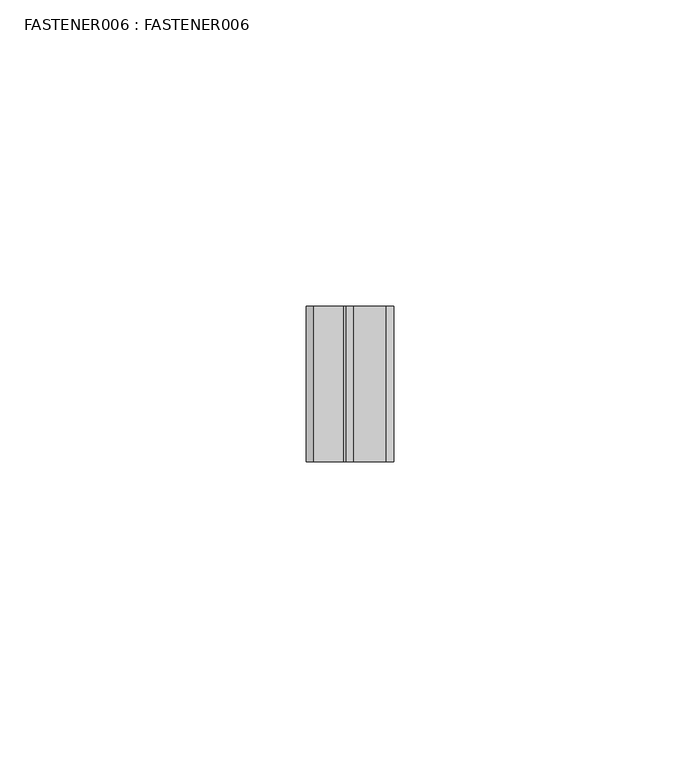
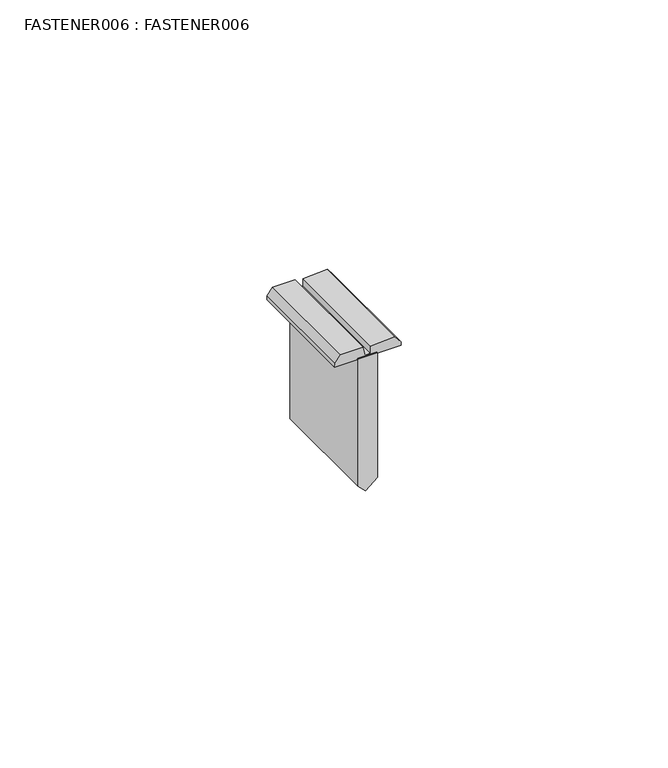
"""IFC4 building model written with IfcOpenShell, lengths in millimetres: proxy geometry, FASTENER006 : FASTENER006."""

import ifcopenshell
import ifcopenshell.guid

model = None  # the IFC model being written
_history = None  # IfcOwnerHistory: only IFC2X3 demands one
_inside = {}  # id of a spatial element -> (the spatial element, [elements in it])
_under = {}  # id of a project, library or spatial element -> (it, [spatial elements below it])
_declared = {}  # id of a project -> (the project, [libraries it declares])
_typed = {}  # id of a type object -> (the type object, [elements of that type])
_made_of = {}  # id of a material, layer set ... -> (it, [elements and type objects made of it])


def new_model(schema):
    """Start an empty IFC model of exactly this schema.

    Asked for "IFC4X3", IfcOpenShell would pick the latest addendum, in which some entities
    have other attributes; the version numbers below select the first issue.
    IFC2X3 requires an IfcOwnerHistory on every rooted entity: one is made here for all.
    """
    global model, _history
    if schema == "IFC4X3":
        model = ifcopenshell.file(schema_version=(4, 3, 0, 0))
    else:
        model = ifcopenshell.file(schema=schema)
    _inside.clear()
    _under.clear()
    _declared.clear()
    _typed.clear()
    _made_of.clear()
    _history = None
    if model.schema == "IFC2X3":
        org = make("IfcOrganization", Name="unknown")
        user = make(
            "IfcPersonAndOrganization",
            ThePerson=make("IfcPerson", FamilyName="unknown"),
            TheOrganization=org,
        )
        app = make(
            "IfcApplication",
            ApplicationDeveloper=org,
            Version="unknown",
            ApplicationFullName="unknown",
            ApplicationIdentifier="unknown",
        )
        _history = make(
            "IfcOwnerHistory",
            OwningUser=user,
            OwningApplication=app,
            ChangeAction="ADDED",
            CreationDate=0,
        )
    return model


def make(cls, **values):
    """One entity of the class cls with the attributes given. An attribute that is None is left unset."""
    return model.create_entity(
        cls, **{name: value for name, value in values.items() if value is not None}
    )


def rooted(cls, **values):
    """An entity with a GlobalId (a new one), such as an element, a storey or a relation."""
    return make(cls, GlobalId=ifcopenshell.guid.new(), OwnerHistory=_history, **values)


def si_unit(unit_type, name, prefix=None):
    """IfcSIUnit, for example si_unit("LENGTHUNIT", "METRE", prefix="MILLI")."""
    return make("IfcSIUnit", UnitType=unit_type, Prefix=prefix, Name=name)


def assignment(units):
    """IfcUnitAssignment: the units of a project."""
    return None if units is None else make("IfcUnitAssignment", Units=units)


def point(xyz):
    """IfcCartesianPoint."""
    return None if xyz is None else make("IfcCartesianPoint", Coordinates=xyz)


def direction(xyz):
    """IfcDirection."""
    return None if xyz is None else make("IfcDirection", DirectionRatios=xyz)


def frame(location, z_axis=None, x_axis=None):
    """IfcAxis2Placement3D, a coordinate frame: its origin and axes. An axis left out is left unset."""
    return make(
        "IfcAxis2Placement3D",
        Location=point(location),
        Axis=direction(z_axis),
        RefDirection=direction(x_axis),
    )


def origin():
    """The frame at (0, 0, 0) with its axes left unset."""
    return frame((0.0, 0.0, 0.0))


def place(relative_to, where):
    """IfcLocalPlacement: puts the frame where relative to a parent placement (None: the world)."""
    return make(
        "IfcLocalPlacement", PlacementRelTo=relative_to, RelativePlacement=where
    )


def context(
    kind, dimensions, precision=None, world=None, true_north=None, identifier=None
):
    """IfcGeometricRepresentationContext, for example the 3D "Model" context."""
    return make(
        "IfcGeometricRepresentationContext",
        ContextIdentifier=identifier,
        ContextType=kind,
        CoordinateSpaceDimension=dimensions,
        Precision=precision,
        WorldCoordinateSystem=world,
        TrueNorth=true_north,
    )


def project(units=None, contexts=None):
    """IfcProject with its units and contexts."""
    return rooted(
        "IfcProject",
        Name="project",
        RepresentationContexts=contexts,
        UnitsInContext=assignment(units),
    )


def spatial(cls, under=None, at=None, **own):
    """A site, building, storey or space (cls), placed at a placement, below another one or the project."""
    s = rooted(cls, ObjectPlacement=at, **own)
    if under is not None:
        _under.setdefault(under.id(), (under, []))[1].append(s)
    return s


def polyline(points):
    """IfcPolyline through the points."""
    return make("IfcPolyline", Points=[point(p) for p in points])


def outline(outer, holes=None, kind="AREA"):
    """IfcArbitraryClosedProfileDef: a profile drawn as a closed curve; with holes, ...WithVoids."""
    if holes is None:
        return make("IfcArbitraryClosedProfileDef", ProfileType=kind, OuterCurve=outer)
    return make(
        "IfcArbitraryProfileDefWithVoids",
        ProfileType=kind,
        OuterCurve=outer,
        InnerCurves=holes,
    )


def extrude(swept, where, along, depth):
    """IfcExtrudedAreaSolid: the profile swept, set in the frame where, extruded along a direction by depth."""
    return make(
        "IfcExtrudedAreaSolid",
        SweptArea=swept,
        Position=where,
        ExtrudedDirection=direction(along),
        Depth=depth,
    )


def shape(context_of_items, identifier, shape_type, items):
    """IfcShapeRepresentation: the items that make up one representation, for example the "Body"."""
    return make(
        "IfcShapeRepresentation",
        ContextOfItems=context_of_items,
        RepresentationIdentifier=identifier,
        RepresentationType=shape_type,
        Items=items,
    )


def source(mapping_origin, context_of_items, identifier, shape_type, items):
    """IfcRepresentationMap: a shape defined once, which mapped items show again and again."""
    return make(
        "IfcRepresentationMap",
        MappingOrigin=mapping_origin,
        MappedRepresentation=shape(context_of_items, identifier, shape_type, items),
    )


def transform(
    local_origin,
    x_axis=None,
    y_axis=None,
    z_axis=None,
    scale=None,
    scale2=None,
    scale3=None,
    uniform=True,
):
    """IfcCartesianTransformationOperator3D, or its non-uniform kind. x_axis, y_axis, z_axis: its Axis1, 2, 3."""
    if uniform:
        return make(
            "IfcCartesianTransformationOperator3D",
            Axis1=direction(x_axis),
            Axis2=direction(y_axis),
            LocalOrigin=point(local_origin),
            Scale=scale,
            Axis3=direction(z_axis),
        )
    return make(
        "IfcCartesianTransformationOperator3DnonUniform",
        Axis1=direction(x_axis),
        Axis2=direction(y_axis),
        LocalOrigin=point(local_origin),
        Scale=scale,
        Axis3=direction(z_axis),
        Scale2=scale2,
        Scale3=scale3,
    )


def mapped(mapping_source, mapping_target):
    """IfcMappedItem: shows the shape of a source again, moved by a transform."""
    return make(
        "IfcMappedItem", MappingSource=mapping_source, MappingTarget=mapping_target
    )


def made_of(thing, what):
    """Note that an element or type object is made of a material, layer set ...; save() writes the relation."""
    if what is not None:
        _made_of.setdefault(what.id(), (what, []))[1].append(thing)
    return thing


def element(
    cls,
    number,
    at=None,
    inside=None,
    cuts=None,
    type_object=None,
    material=None,
    context=None,
    identifier="Body",
    shape_type=None,
    held_by="IfcProductDefinitionShape",
    body=None,
    shapes=None,
    **own,
):
    """One element of the class cls, such as IfcWall. Its Tag is "e" and its number.

    at: its placement. inside: the storey or other place that contains it. cuts: it is an
    opening in that element (IfcRelVoidsElement). A single representation is given by context,
    identifier, shape_type and body (its items); several are given by shapes. held_by: the class
    of the entity that holds the representations. save() writes the other relations.
    """
    e = rooted(cls, Tag="e%d" % number, ObjectPlacement=at, **own)
    if body is not None:
        shapes = [shape(context, identifier, shape_type, body)]
    if shapes is not None:
        e.Representation = make(held_by, Representations=shapes)
    if inside is not None:
        _inside.setdefault(inside.id(), (inside, []))[1].append(e)
    if cuts is not None:
        rooted(
            "IfcRelVoidsElement", RelatingBuildingElement=cuts, RelatedOpeningElement=e
        )
    if type_object is not None:
        _typed.setdefault(type_object.id(), (type_object, []))[1].append(e)
    return made_of(e, material)


def aggregate(whole, parts):
    """IfcRelAggregates: a whole, such as a stair, and the parts it consists of."""
    return rooted("IfcRelAggregates", RelatingObject=whole, RelatedObjects=parts)


def save(model, path):
    """Write the relations noted so far, then the file.

    IfcRelAggregates (storeys below a building ...), IfcRelContainedInSpatialStructure (elements
    in a storey), IfcRelDefinesByType, IfcRelAssociatesMaterial and IfcRelDeclares: one each for
    every whole, place, type object, material and project.
    """
    for whole, parts in _under.values():
        aggregate(whole, parts)
    for where, things in _inside.values():
        rooted(
            "IfcRelContainedInSpatialStructure",
            RelatedElements=things,
            RelatingStructure=where,
        )
    for kind, things in _typed.values():
        rooted("IfcRelDefinesByType", RelatedObjects=things, RelatingType=kind)
    for what, things in _made_of.values():
        rooted("IfcRelAssociatesMaterial", RelatedObjects=things, RelatingMaterial=what)
    for by, libraries in _declared.values():
        rooted("IfcRelDeclares", RelatingContext=by, RelatedDefinitions=libraries)
    model.write(path)


def fastener006_fastener006_f031ca55(model_context):
    return source(origin(), model_context, "Body", "SweptSolid", [
        extrude(outline(polyline([(42577.1576024, 5870.6890035), (42548.1988623, 5870.6890035), (42546.5833096, 5872.3460181), (42548.7638676, 5874.895922), (42577.1576024, 5874.895922), (42577.1576024, 5870.6890035)])), frame((0.0, -1078.2906574, 0.0), z_axis=(0.0, 1.0, 0.0), x_axis=(0.0, 0.0, 1.0)), (0.0, 0.0, 1.0), 25.4),
        extrude(outline(polyline([(42577.1576024, 5879.9417891), (42577.9674245, 5879.9417891), (42579.5612959, 5878.7030871), (42579.1650604, 5873.4174049), (42577.5756297, 5873.4174049), (42577.5756297, 5872.1703), (42579.587761, 5871.7740645), (42579.587761, 5866.8949826), (42577.9938896, 5865.6562805), (42577.1576024, 5865.6454839), (42577.1576024, 5879.9417891)])), frame((0.0, -1078.2906574, 0.0), z_axis=(0.0, 1.0, 0.0), x_axis=(0.0, 0.0, 1.0)), (0.0, 0.0, 1.0), 25.4),
    ])


if __name__ == "__main__":
    model = new_model("IFC4")
    model_context = context("Model", 3, world=origin())
    ifc_project = project(units=[si_unit("LENGTHUNIT", "METRE", prefix="MILLI")], contexts=[model_context])
    site = spatial("IfcSite", under=ifc_project)
    building = spatial("IfcBuilding", under=site)
    placement = place(None, origin())
    fastener006_fastener006_shape = fastener006_fastener006_f031ca55(model_context)
    element("IfcBuildingElementProxy", 1, Name="FASTENER006 : FASTENER006", ObjectType="FASTENER006 : FASTENER006", at=placement, inside=building, context=model_context, shape_type="MappedRepresentation", body=[
        mapped(fastener006_fastener006_shape, transform((0.0, 0.0, 0.0), x_axis=(1.0, 0.0, 0.0), y_axis=(0.0, 1.0, 0.0), z_axis=(0.0, 0.0, 1.0))),
    ])
    save(model, "model.ifc")

# Revit data of these elements
# Type "FASTENER006 : FASTENER006"
#   NameOverride = "FASTENER006"
# Element 1 (IfcBuildingElementProxy, "FASTENER006 : FASTENER006")
#   Materials on its faces: "ENGINEERED PANCAKE HEAD FASTENER @ 12\" O.C."
# Materials
#   "ENGINEERED PANCAKE HEAD FASTENER @ 12\" O.C.": class "Unassigned", colour RGB 255 255 255, transparency 0, Cost = 0
